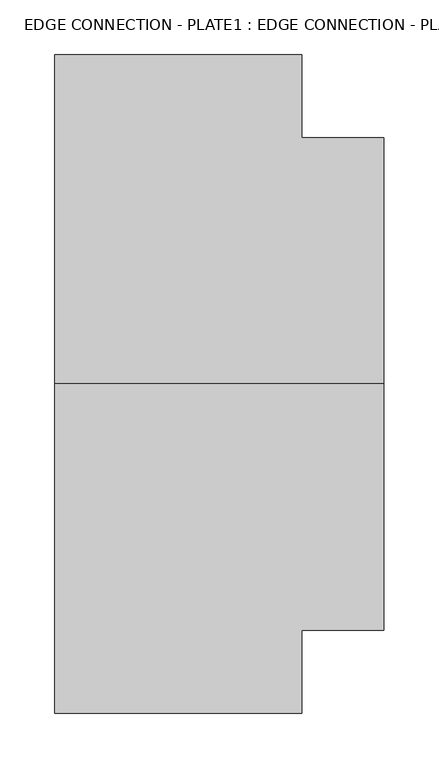
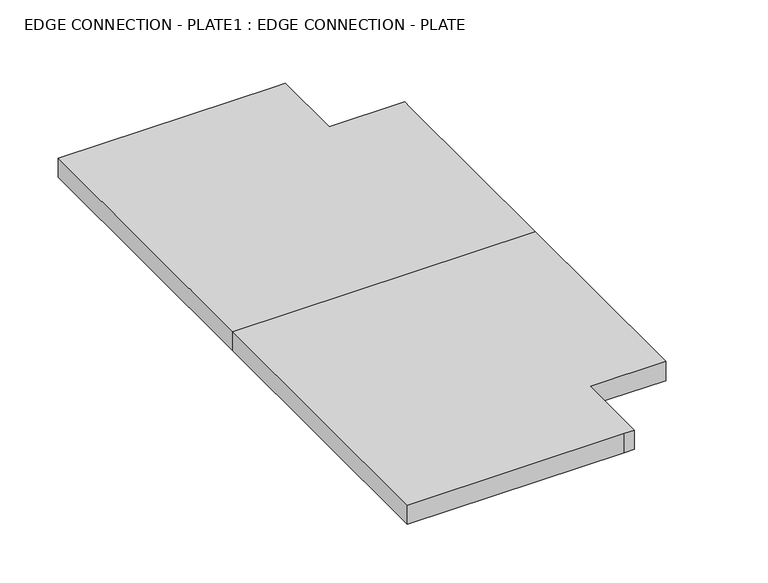
"""IFC4 building model written with IfcOpenShell, lengths in millimetres: fastener geometry, EDGE CONNECTION - PLATE1 : EDGE CONNECTION - PLATE."""

from ifc_helpers import new_model, si_unit, frame, origin, place, context, project, spatial, polyline, outline, extrude, source, transform, mapped, element, save


def edge_connection_plate1_edge_connection_plate_36d6623d(model_context):
    return source(origin(), model_context, "Body", "SweptSolid", [
        extrude(outline(polyline([(300.0, 22499.5208589), (300.0, 22285.0508589), (300.0, 22275.0508589), (225.138, 22275.0508589), (225.138, 22199.5208589), (215.138, 22199.5208589), (0.0, 22199.5208589), (0.0, 22499.5208589), (300.0, 22499.5208589)])), frame((0.0, 0.0, 200.0), z_axis=(0.0, 0.0, 1.0), x_axis=(1.0, 0.0, 0.0)), (0.0, 0.0, 1.0), 20.0),
        extrude(outline(polyline([(300.0, 22499.5208589), (0.0, 22499.5208589), (0.0, 22799.5208589), (215.138, 22799.5208589), (225.138, 22799.5208589), (225.138, 22723.9908589), (300.0, 22723.9908589), (300.0, 22713.9908589), (300.0, 22499.5208589)])), frame((0.0, 0.0, 200.0), z_axis=(0.0, 0.0, 1.0), x_axis=(1.0, 0.0, 0.0)), (0.0, 0.0, 1.0), 20.0),
    ])


if __name__ == "__main__":
    model = new_model("IFC4")
    model_context = context("Model", 3, world=origin())
    ifc_project = project(units=[si_unit("LENGTHUNIT", "METRE", prefix="MILLI")], contexts=[model_context])
    site = spatial("IfcSite", under=ifc_project)
    building = spatial("IfcBuilding", under=site)
    placement = place(None, origin())
    edge_connection_plate1_edge_connection_plate_shape = edge_connection_plate1_edge_connection_plate_36d6623d(model_context)
    element("IfcFastener", 1, ObjectType="EDGE CONNECTION - PLATE1 : EDGE CONNECTION - PLATE", at=placement, inside=building, context=model_context, shape_type="MappedRepresentation", body=[
        mapped(edge_connection_plate1_edge_connection_plate_shape, transform((0.0, 0.0, 0.0), x_axis=(1.0, 0.0, 0.0), y_axis=(0.0, 1.0, 0.0), z_axis=(0.0, 0.0, 1.0))),
    ])
    save(model, "model.ifc")
